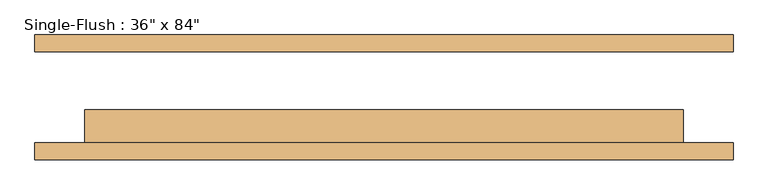
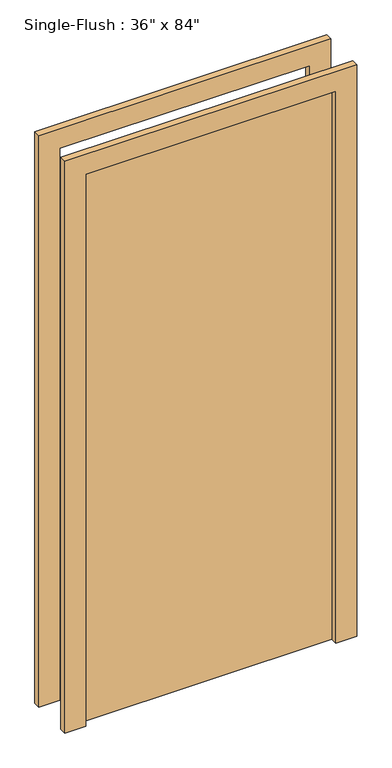
"""IFC4 building model written with IfcOpenShell, lengths in millimetres: door geometry."""

from ifc_helpers import new_model, si_unit, frame, origin, origin_with_axes, place, context, project, spatial, polyline, outline, extrude, source, transform, mapped, element, save


def door_9814c99b(model_context):
    return source(origin(), model_context, "Body", "SweptSolid", [
        extrude(outline(polyline([(2209.8, -533.4), (0.0, -533.4), (0.0, -457.2), (2133.6, -457.2), (2133.6, 457.2), (0.0, 457.2), (0.0, 533.4), (2209.8, 533.4), (2209.8, -533.4)])), frame((0.0, -95.25, 0.0), z_axis=(0.0, 1.0, 0.0), x_axis=(0.0, 0.0, 1.0)), (0.0, 0.0, 1.0), 25.4),
        extrude(outline(polyline([(2209.8, 533.4), (2209.8, -533.4), (0.0, -533.4), (0.0, -457.2), (2133.6, -457.2), (2133.6, 457.2), (0.0, 457.2), (0.0, 533.4), (2209.8, 533.4)])), frame((0.0, 69.85, 0.0), z_axis=(0.0, 1.0, 0.0), x_axis=(0.0, 0.0, 1.0)), (0.0, 0.0, 1.0), 25.4),
        extrude(outline(polyline([(457.2, -19.05), (457.2, -69.85), (-457.2, -69.85), (-457.2, -19.05), (457.2, -19.05)])), origin_with_axes(), (0.0, 0.0, 1.0), 2133.6),
    ])


if __name__ == "__main__":
    model = new_model("IFC4")
    model_context = context("Model", 3, world=origin())
    ifc_project = project(units=[si_unit("LENGTHUNIT", "METRE", prefix="MILLI")], contexts=[model_context])
    site = spatial("IfcSite", under=ifc_project)
    building = spatial("IfcBuilding", under=site)
    placement = place(None, origin())
    door_shape = door_9814c99b(model_context)
    element("IfcDoor", 1, ObjectType="Single-Flush : 36\" x 84\"", at=placement, inside=building, context=model_context, shape_type="MappedRepresentation", body=[
        mapped(door_shape, transform((0.0, 0.0, 0.0), x_axis=(1.0, 0.0, 0.0), y_axis=(0.0, 1.0, 0.0), z_axis=(0.0, 0.0, 1.0))),
    ])
    save(model, "model.ifc")

# Revit data of these elements
# Type "Single-Flush : 36\" x 84\""
#   Type Mark = "29"
#   Assembly Code = "C1020"
#   Thickness = 0' - 2"
#   Height = 7' - 0"
#   Trim Projection Ext = 0' - 1"
#   Trim Projection Int = 0' - 1"
#   Trim Width = 0' - 3"
#   Width = 3' - 0"
#   Function = 0
#   Door Material = Door - Panel
#   Frame Material = Concrete - Cast-in-Place Concrete
#   Wall Closure = (empty or 0)
# Element 1 (IfcDoor, "Single-Flush : 36\" x 84\"")
#   Materials on its faces: "Concrete - Cast-in-Place Concrete", "Door - Panel"
# Materials
#   "Door - Panel": class "Wood", colour RGB 149 143 132, transparency 0, Comments = "Rendering appearance not upgraded Rendering appearance not upgraded "
#   "Concrete - Cast-in-Place Concrete": class "Concrete", colour RGB 178 178 178, transparency 0, Comments = "Rendering appearance not upgraded Rendering appearance not upgraded ", Description = "Concrete"
